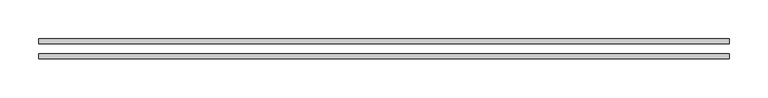
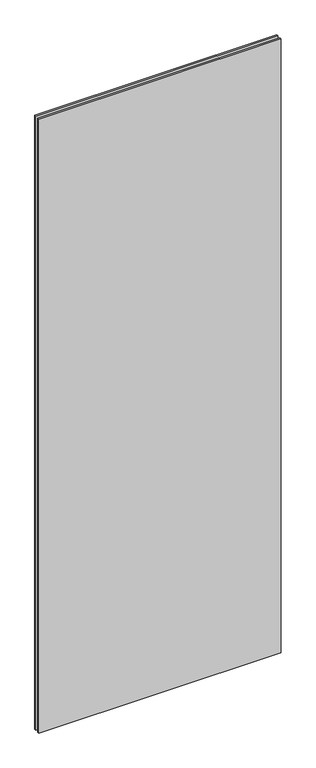
"""IFC4 building model written with IfcOpenShell, lengths in millimetres: proxy geometry, Window glass:Window glass:300352:Window glass:300352 : Window glass:Window glass:300352:300073:Window glass:300352:Window glass:300352 : Window glass:Window glass:300352:300073 : Window glass:Window glass:300352:Window glass:300352 : Window glass:Window glass:300352:300073:3 : Window glass:Window glass:300352:Window glass:300352 : Window glass:Window glass:300352:300073:Window glass:300352:Window glass:300352 : Window glass:Window glass:300352:300073 : Window glass:Window glass:300352:Window glass:300352 : Window glass:Window glass:300352:300073:300061."""

from ifc_helpers import new_model, si_unit, frame, origin, place, context, project, spatial, polyline, outline, extrude, source, transform, mapped, element, save


def generic_models_ed74a05d(model_context):
    return source(origin(), model_context, "Body", "SweptSolid", [
        extrude(outline(polyline([(570404.7161787, -579048.3332724), (569517.8947692, -579048.3332724), (569517.8947692, -579041.9832724), (570404.7161787, -579041.9832724), (570404.7161787, -579048.3332724)])), frame((0.0, 0.0, 71.8093465), z_axis=(0.0, 0.0, 1.0), x_axis=(1.0, 0.0, 0.0)), (0.0, 0.0, 1.0), 2375.862329),
        extrude(outline(polyline([(570404.7161787, -579029.2832724), (569517.8947692, -579029.2832724), (569517.8947692, -579022.9332724), (570404.7161787, -579022.9332724), (570404.7161787, -579029.2832724)])), frame((0.0, 0.0, 71.8093465), z_axis=(0.0, 0.0, 1.0), x_axis=(1.0, 0.0, 0.0)), (0.0, 0.0, 1.0), 2375.862329),
    ])


if __name__ == "__main__":
    model = new_model("IFC4")
    model_context = context("Model", 3, world=origin())
    ifc_project = project(units=[si_unit("LENGTHUNIT", "METRE", prefix="MILLI")], contexts=[model_context])
    site = spatial("IfcSite", under=ifc_project)
    building = spatial("IfcBuilding", under=site)
    placement = place(None, origin())
    generic_models_shape = generic_models_ed74a05d(model_context)
    element("IfcBuildingElementProxy", 1, Name="Window glass:Window glass:300352:Window glass:300352 : Window glass:Window glass:300352:300073:Window glass:300352:Window glass:300352 : Window glass:Window glass:300352:300073 : Window glass:Window glass:300352:Window glass:300352 : Window glass:Window glass:300352:300073:3 : Window glass:Window glass:300352:Window glass:300352 : Window glass:Window glass:300352:300073:Window glass:300352:Window glass:300352 : Window glass:Window glass:300352:300073 : Window glass:Window glass:300352:Window glass:300352 : Window glass:Window glass:300352:300073:300061", ObjectType="Window glass:Window glass:300352:Window glass:300352 : Window glass:Window glass:300352:300073:Window glass:300352:Window glass:300352 : Window glass:Window glass:300352:300073 : Window glass:Window glass:300352:Window glass:300352 : Window glass:Window glass:300352:300073:3 : Window glass:Window glass:300352:Window glass:300352 : Window glass:Window glass:300352:300073:Window glass:300352:Window glass:300352 : Window glass:Window glass:300352:300073 : Window glass:Window glass:300352:Window glass:300352 : Window glass:Window glass:300352:300073:300061", at=placement, inside=building, context=model_context, shape_type="MappedRepresentation", body=[
        mapped(generic_models_shape, transform((0.0, 0.0, 0.0), x_axis=(1.0, 0.0, 0.0), y_axis=(0.0, 1.0, 0.0), z_axis=(0.0, 0.0, 1.0))),
    ])
    save(model, "model.ifc")

# Revit data of these elements
# Type "Window glass:Window glass:300352:Window glass:300352 : Window glass:Window glass:300352:300073:Window glass:300352:Window glass:300352 : Window glass:Window glass:300352:300073 : Window glass:Window glass:300352:Window glass:300352 : Window glass:Window glass:300352:300073:3 : Window glass:Window glass:300352:Window glass:300352 : Window glass:Window glass:300352:300073:Window glass:300352:Window glass:300352 : Window glass:Window glass:300352:300073 : Window glass:Window glass:300352:Window glass:300352 : Window glass:Window glass:300352:300073:300061"
#   NameOverride = "Window glass:Window glass:300352:Window glass:300352 : Window glass:Window glass:300352:300073:Window glass:300352:Window glass:300352 : Window glass:Window glass:300352:300073 : Window glass:Window glass:300352:Window glass:300352 : Window glass:Window glass:300352:300073:300061"
#   ObjectTypeOverride = "Window glass:300352:Window glass:300352 : Window glass:Window glass:300352:300073 : Window glass:Window glass:300352:Window glass:300352 : Window glass:Window glass:300352:300073"
#   Reference = "Window glass"
#   Tag = "300061"
# Element 1 (IfcBuildingElementProxy, "Window glass:Window glass:300352:Window glass:300352 : Window glass:Window glass:300352:300073:Window glass:300352:Window glass:300352 : Window glass:Window glass:300352:300073 : Window glass:Window glass:300352:Window glass:300352 : Window glass:Window glass:300352:300073:3 : Window glass:Window glass:300352:Window glass:300352 : Window glass:Window glass:300352:300073:Window glass:300352:Window glass:300352 : Window glass:Window glass:300352:300073 : Window glass:Window glass:300352:Window glass:300352 : Window glass:Window glass:300352:300073:300061")
#   Materials on its faces: "INSULATED LOW-E GLAZING (SEE ELEVATIONS FOR U-FACTOR, SHGC, & LT)"
# Materials
#   "INSULATED LOW-E GLAZING (SEE ELEVATIONS FOR U-FACTOR, SHGC, & LT)": class "Unassigned", colour RGB 84 171 255, transparency 0, Cost = 0
